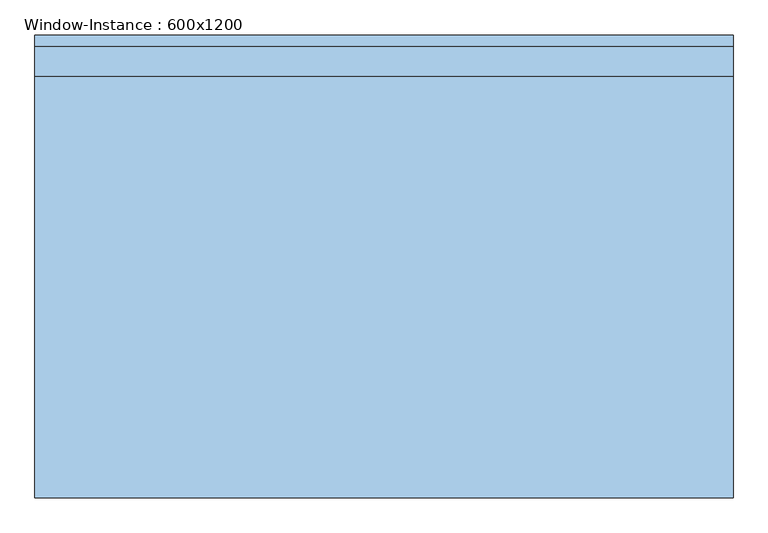
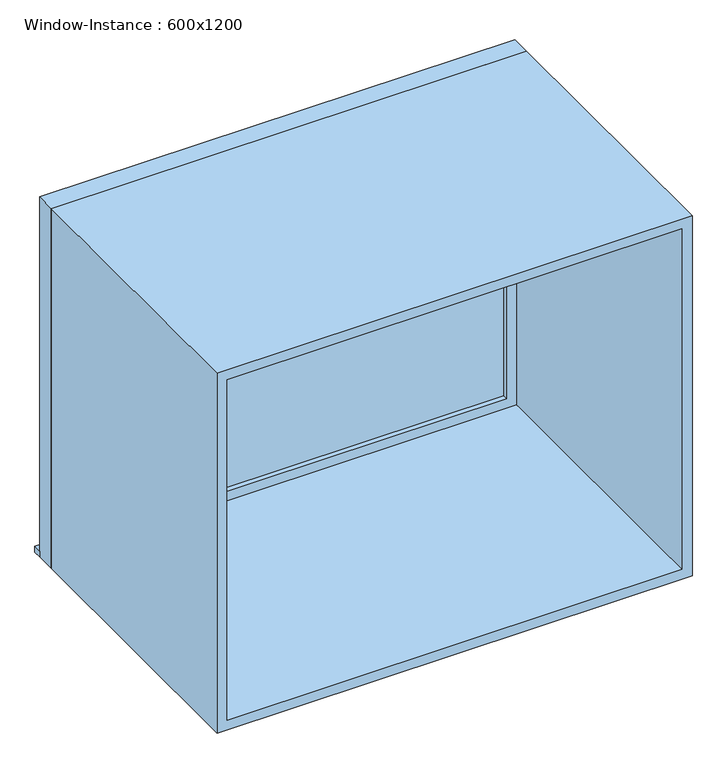
"""IFC4 building model written with IfcOpenShell, lengths in millimetres: window geometry, Window-Instance : 600x1200."""

from ifc_helpers import new_model, si_unit, frame, origin, place, context, project, spatial, polyline, outline, extrude, source, transform, mapped, element, save


def window_instance_600x1200_499b88cb(model_context):
    return source(origin(), model_context, "Body", "SweptSolid", [
        extrude(outline(polyline([(-788.1, 510.4), (711.9, 510.4), (711.9, 485.0), (-788.1, 485.0), (-788.1, 510.4)])), frame((0.0, 0.0, 900.0), z_axis=(0.0, 0.0, 1.0), x_axis=(1.0, 0.0, 0.0)), (0.0, 0.0, 1.0), 19.05),
        extrude(outline(polyline([(648.4, 436.425), (-724.6, 436.425), (-724.6, 449.125), (648.4, 449.125), (648.4, 436.425)])), frame((0.0, 0.0, 963.5), z_axis=(0.0, 0.0, 1.0), x_axis=(1.0, 0.0, 0.0)), (0.0, 0.0, 1.0), 1073.0),
        extrude(outline(polyline([(2080.95, -769.05), (919.05, -769.05), (919.05, 692.85), (2080.95, 692.85), (2080.95, -769.05)]), holes=[polyline([(2036.5, -724.6), (2036.5, 648.4), (963.5, 648.4), (963.5, -724.6), (2036.5, -724.6)])]), frame((0.0, 420.55, 0.0), z_axis=(0.0, 1.0, 0.0), x_axis=(0.0, 0.0, 1.0)), (0.0, 0.0, 1.0), 44.45),
        extrude(outline(polyline([(2100.0, -788.1), (900.0, -788.1), (900.0, 711.9), (2100.0, 711.9), (2100.0, -788.1)]), holes=[polyline([(2068.25, -756.35), (2068.25, 680.15), (931.75, 680.15), (931.75, -756.35), (2068.25, -756.35)])]), frame((0.0, -485.0, 0.0), z_axis=(0.0, 1.0, 0.0), x_axis=(0.0, 0.0, 1.0)), (0.0, 0.0, 1.0), 905.55),
        extrude(outline(polyline([(2100.0, 711.9), (2100.0, -788.1), (900.0, -788.1), (900.0, 711.9), (2100.0, 711.9)]), holes=[polyline([(2080.95, 692.85), (919.05, 692.85), (919.05, -769.05), (2080.95, -769.05), (2080.95, 692.85)])]), frame((0.0, 420.55, 0.0), z_axis=(0.0, 1.0, 0.0), x_axis=(0.0, 0.0, 1.0)), (0.0, 0.0, 1.0), 64.45),
    ])


if __name__ == "__main__":
    model = new_model("IFC4")
    model_context = context("Model", 3, world=origin())
    ifc_project = project(units=[si_unit("LENGTHUNIT", "METRE", prefix="MILLI")], contexts=[model_context])
    site = spatial("IfcSite", under=ifc_project)
    building = spatial("IfcBuilding", under=site)
    placement = place(None, origin())
    window_instance_600x1200_shape = window_instance_600x1200_499b88cb(model_context)
    element("IfcWindow", 1, ObjectType="Window-Instance : 600x1200", at=placement, inside=building, context=model_context, shape_type="MappedRepresentation", body=[
        mapped(window_instance_600x1200_shape, transform((0.0, 0.0, 0.0), x_axis=(1.0, 0.0, 0.0), y_axis=(0.0, 1.0, 0.0), z_axis=(0.0, 0.0, 1.0))),
    ])
    save(model, "model.ifc")

# Revit data of these elements
# Type "Window-Instance : 600x1200"
#   Type Mark = "7"
#   Construction Type Id = "GSP4R"
#   Assembly Code = "B2020100"
#   Analytic Construction = "1/8 in Pilkington single glazing"
#   Visual Light Transmittance = 0.9
#   Thermal Resistance (R) = 0.149095 (m²·K)/W
#   Solar Heat Gain Coefficient = 0.86
#   Heat Transfer Coefficient (U) = 6.70716 W/(m²·K)
#   Height [instance default] = 1200 mm
#   Default Sill Height = 900 mm
#   Width [instance default] = 600 mm
#   Window Inset = 20 mm
#   Glass Pane Material = WW-EC-GL-Storefront
#   Sash Material = WW-EC-RGB-White
#   Wall Closure = (empty or 0)
# Element 1 (IfcWindow, "Window-Instance : 600x1200")
#   Width = 1500 mm
#   Materials on its faces: "WW-EC-RGB-White", "WW-EC-GL-Storefront"
# Materials
#   "WW-EC-GL-Storefront": class "Glass", colour RGB 236 240 239, transparency 0.85, Description = "Storefront Glass", Cost = 0
#   "WW-EC-RGB-White": class "Generic", colour RGB 255 255 255, transparency 0, Comments = "If region requests off-white, swith asset color to RGB 231-228-220", Description = "Generic Color", Cost = 0
